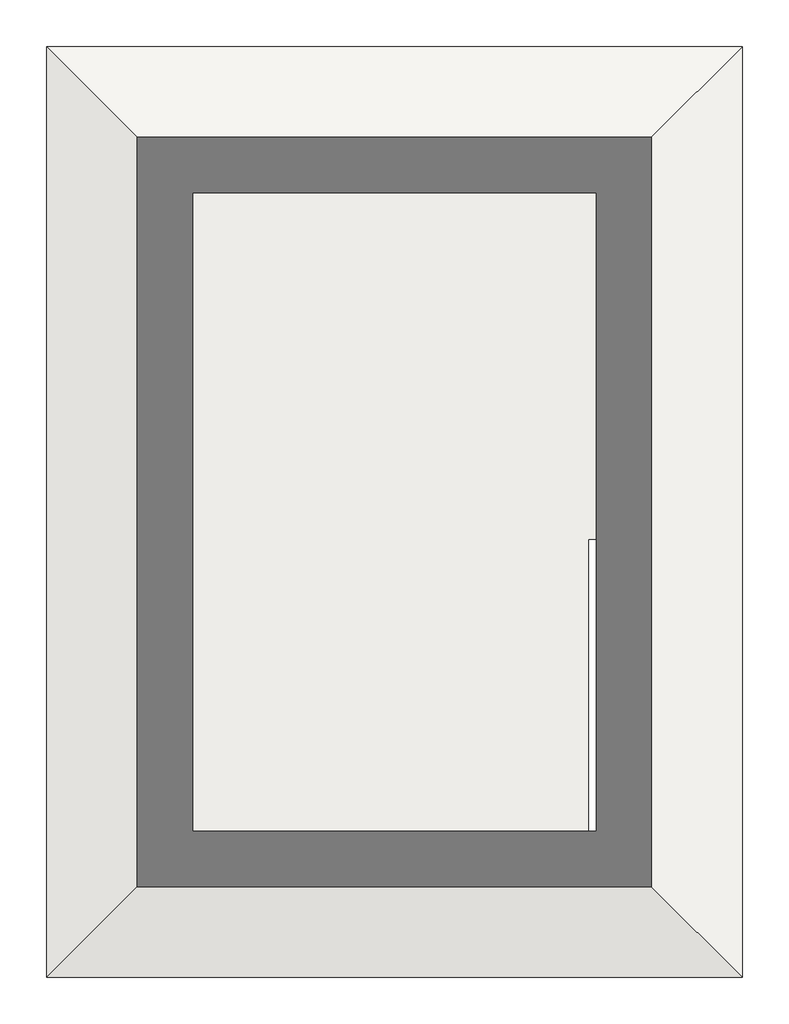
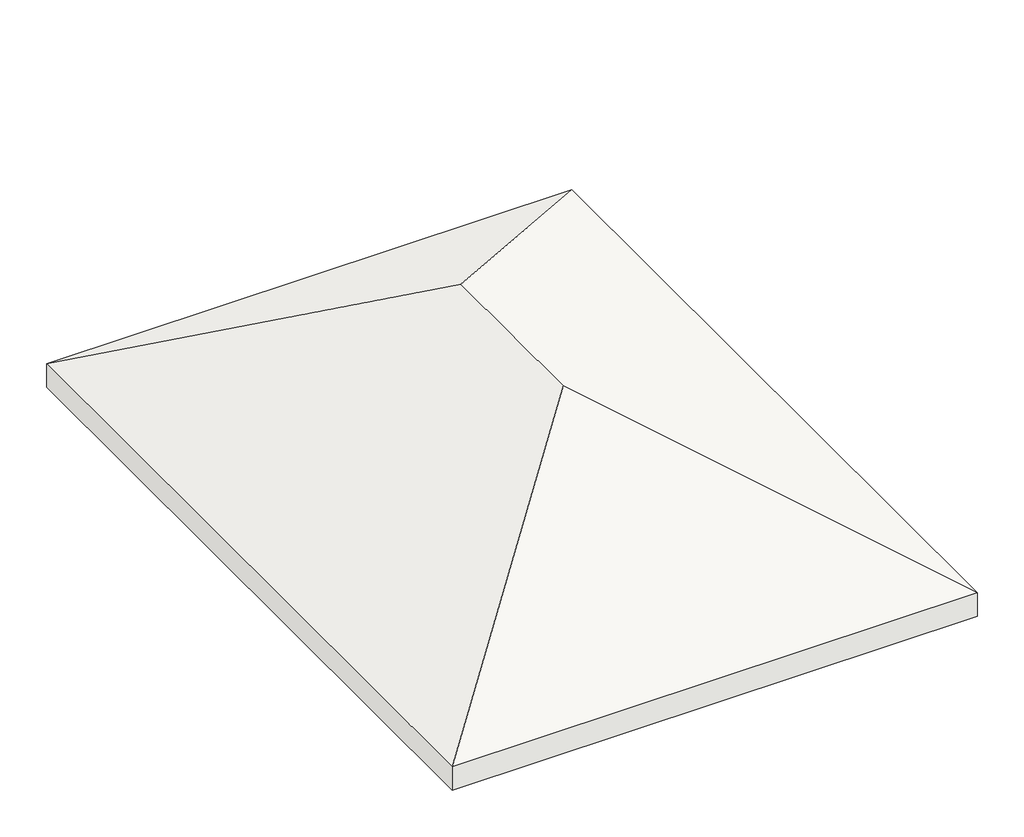
# One storey: 4 walls, 1 roof, 1 slab.
"""IFC4 building model written with IfcOpenShell, lengths in millimetres."""

from ifc_helpers import new_model, si_unit, frame, origin, place, context, project, spatial, polyline, outline, extrude, faceted_brep, element, save

model = new_model("IFC4")

# Units and contexts
model_context = context("Model", 3, world=origin())
ifc_project = project(units=[si_unit("LENGTHUNIT", "METRE", prefix="MILLI")], contexts=[model_context])

# Site, building, storey
site = spatial("IfcSite", under=ifc_project)
building = spatial("IfcBuilding", under=site)
storey = spatial("IfcBuildingStorey", under=building, Name="Уровень 4", Elevation=8400.0)

# Roof
placement = place(None, origin())
element("IfcRoof", 1, ObjectType="Типовой - 400мм", at=placement, inside=storey, context=model_context, shape_type="Brep", body=[
    faceted_brep([(-14630.6631644, -9504.3393422, 11249.2235785), (-9695.6631644, -14439.3393422, 8400.0), (-19565.6631644, -14439.3393422, 8400.0), (-19565.6631644, -1239.3393422, 8400.0), (-14630.6631644, -6174.3393422, 11249.2235785), (-9695.6631644, -1239.3393422, 8400.0), (-9695.6631644, -14439.3393422, 8861.8802154), (-14630.6631644, -9504.3393422, 11711.1037938), (-19565.6631644, -14439.3393422, 8861.8802154), (-19565.6631644, -1239.3393422, 8861.8802154), (-14630.6631644, -6174.3393422, 11711.1037938), (-9695.6631644, -1239.3393422, 8861.8802154)], [[[0, 1, 2]], [[3, 4, 0, 2]], [[5, 4, 3]], [[1, 0, 4, 5]], [[6, 7, 8]], [[9, 8, 7, 10]], [[11, 9, 10]], [[6, 11, 10, 7]], [[5, 11, 6, 1]], [[3, 9, 11, 5]], [[2, 8, 9, 3]], [[1, 6, 8, 2]]]),
])

# Slab
element("IfcSlab", 2, ObjectType="Монолитный бетон 225мм", at=placement, inside=storey, context=model_context, shape_type="SweptSolid", body=[
    extrude(outline(polyline([(-18880.6631644, -13322.3774925), (-18880.6631644, -2222.3774925), (-10380.6631644, -2222.3774925), (-10380.6631644, -8222.3774925), (-11880.6631644, -8222.3774925), (-11880.6631644, -13322.3774925), (-18880.6631644, -13322.3774925)])), frame((0.0, 0.0, 8395.0), z_axis=(0.0, 0.0, 1.0), x_axis=(1.0, 0.0, 0.0)), (0.0, 0.0, 1.0), 225.0),
])

# Walls
element("IfcWall", 3, ObjectType="Типовой - Кладка 370 мм", at=placement, inside=storey, context=model_context, shape_type="Brep", body=[
    faceted_brep([(-19065.6631644, -2037.3774925, 8400.0), (-19065.6631644, -13507.3774925, 8400.0), (-19065.6631644, -13507.3774925, 8688.6751346), (-19065.6631644, -2037.3774925, 8688.6751346), (-18695.6631644, -2037.3774925, 8400.0), (-18695.6631644, -2037.3774925, 8860.7475409), (-18695.6631644, -2109.3393422, 8902.2947342), (-18695.6631644, -2407.3774925, 8902.2947342), (-18695.6631644, -13137.3774925, 8902.2947342), (-18695.6631644, -13507.3774925, 8902.2947342), (-18695.6631644, -13507.3774925, 8400.0), (-18695.6631644, -13137.3774925, 8400.0), (-18695.6631644, -2407.3774925, 8400.0), (-18767.6250141, -2037.3774925, 8860.7475409)], [[[0, 1, 2, 3]], [[4, 5, 6, 7, 8, 9, 10, 11, 12]], [[1, 0, 4, 12, 11, 10]], [[2, 1, 10, 9]], [[0, 3, 13, 5, 4]], [[3, 2, 9, 8, 7, 6, 13]], [[6, 5, 13]]]),
])
element("IfcWall", 4, ObjectType="Типовой - Кладка 370 мм", at=placement, inside=storey, context=model_context, shape_type="Brep", body=[
    faceted_brep([(-18695.6631644, -13507.3774925, 8400.0), (-10195.6631644, -13507.3774925, 8400.0), (-10195.6631644, -13507.3774925, 8688.6751346), (-10627.6250141, -13507.3774925, 8938.0684248), (-18633.7013147, -13507.3774925, 8938.0684248), (-18695.6631644, -13507.3774925, 8902.2947342), (-18695.6631644, -13137.3774925, 8400.0), (-18695.6631644, -13137.3774925, 8902.2947342), (-18263.7013147, -13137.3774925, 9151.6880244), (-10997.6250141, -13137.3774925, 9151.6880244), (-10565.6631644, -13137.3774925, 8902.2947342), (-10195.6631644, -13137.3774925, 8688.6751346), (-10195.6631644, -13137.3774925, 8400.0), (-10565.6631644, -13137.3774925, 8400.0)], [[[0, 1, 2, 3, 4, 5]], [[6, 7, 8, 9, 10, 11, 12, 13]], [[1, 0, 6, 13, 12]], [[0, 5, 7, 6]], [[2, 1, 12, 11]], [[5, 4, 8, 7]], [[4, 3, 9, 8]], [[3, 2, 11, 10, 9]]]),
])
element("IfcWall", 5, ObjectType="Типовой - Кладка 370 мм", at=placement, inside=storey, context=model_context, shape_type="Brep", body=[
    faceted_brep([(-10195.6631644, -13137.3774925, 8400.0), (-10195.6631644, -2037.3774925, 8400.0), (-10195.6631644, -2037.3774925, 8688.6751346), (-10195.6631644, -13137.3774925, 8688.6751346), (-10565.6631644, -13137.3774925, 8400.0), (-10565.6631644, -13137.3774925, 8902.2947342), (-10565.6631644, -2407.3774925, 8902.2947342), (-10565.6631644, -2109.3393422, 8902.2947342), (-10565.6631644, -2037.3774925, 8860.7475409), (-10565.6631644, -2037.3774925, 8400.0), (-10565.6631644, -2407.3774925, 8400.0), (-10493.7013147, -2037.3774925, 8860.7475409)], [[[0, 1, 2, 3]], [[4, 5, 6, 7, 8, 9, 10]], [[1, 0, 4, 10, 9]], [[0, 3, 5, 4]], [[2, 1, 9, 8, 11]], [[3, 2, 11, 7, 6, 5]], [[11, 8, 7]]]),
])
element("IfcWall", 6, ObjectType="Типовой - Кладка 370 мм", at=placement, inside=storey, context=model_context, shape_type="Brep", body=[
    faceted_brep([(-10565.6631644, -2037.3774925, 8400.0), (-18695.6631644, -2037.3774925, 8400.0), (-18695.6631644, -2037.3774925, 8860.7475409), (-10565.6631644, -2037.3774925, 8860.7475409), (-10565.6631644, -2407.3774925, 8400.0), (-10565.6631644, -2407.3774925, 8902.2947342), (-10863.7013147, -2407.3774925, 9074.3671405), (-18397.6250141, -2407.3774925, 9074.3671405), (-18695.6631644, -2407.3774925, 8902.2947342), (-18695.6631644, -2407.3774925, 8400.0), (-18695.6631644, -2109.3393422, 8902.2947342), (-10565.6631644, -2109.3393422, 8902.2947342)], [[[0, 1, 2, 3]], [[4, 5, 6, 7, 8, 9]], [[1, 0, 4, 9]], [[2, 1, 9, 8, 10]], [[0, 3, 11, 5, 4]], [[3, 2, 10, 7, 6, 11]], [[10, 8, 7]], [[6, 5, 11]]]),
])

save(model, "model.ifc")

# Revit data of these elements
# Type "Типовой - 400мм"
#   Layers, outside or top first: 400 mm no material (function 1)
# Type "Монолитный бетон 225мм"
#   Function = 0
#   Layers, outside or top first: 50 mm "Бетон, брус для разравнивания песка/цемента" (function 1); 0 mm "Гидроизоляция" (function 100); 175 mm "Бетон, монолитный" (function 1)
# Type "Типовой - Кладка 370 мм"
#   Layers, outside or top first: 370 mm "Бетонные модули для кладки" (function 1)
# Element 1 (IfcRoof, "Типовой - 400мм")
#   built-in parameter 1001705 = 38.4223 (stored number, unit not read)
#   built-in parameter 1001710 = 33615
#   Phase Created = Новая конструкция
#   Materials on its faces: "Крыша по умолчанию"
# Element 2 (IfcSlab, "Монолитный бетон 225мм")
#   built-in parameter 1001955 = -1.5708 (stored number, unit not read)
#   Height Offset From Level = 220 mm
#   Phase Created = Новая конструкция
#   Materials on its faces: "Бетон, монолитный", "Бетон, брус для разравнивания песка/цемента"
# Elements 3, 4, 5, 6 (IfcWall, "Типовой - Кладка 370 мм")
#   Top Offset = 0 mm
#   Base Offset = 0 mm
#   Unconnected Height = 500 mm
#   wall height = 500 mm
#   Phase Created = Новая конструкция
#   Base Constraint = Уровень 4
#   Materials on its faces: "Бетонные модули для кладки"
# Materials
#   "Бетон, брус для разравнивания песка/цемента": class "Бетон", colour RGB 127 127 127, transparency 0, Description = "Покрытие бетонной плиты", Cost = 0
#   "Гидроизоляция": class "Типовой", colour RGB 127 127 127, transparency 0, Description = "Гидроизоляция", Cost = 0
#   "Бетон, монолитный": class "Бетон", colour RGB 192 192 192, transparency 0, Description = "физический материал", Cost = 0
#   "Бетонные модули для кладки": class "Кладка", colour RGB 181 181 181, transparency 0, Description = "Бетонные модули для кладки", Cost = 0
#   "Крыша по умолчанию": class "Разное", colour RGB 0 127 0, transparency 0, Cost = 0
